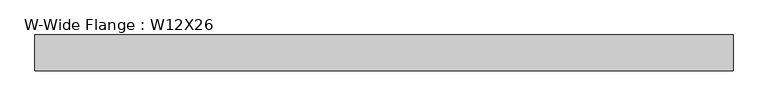
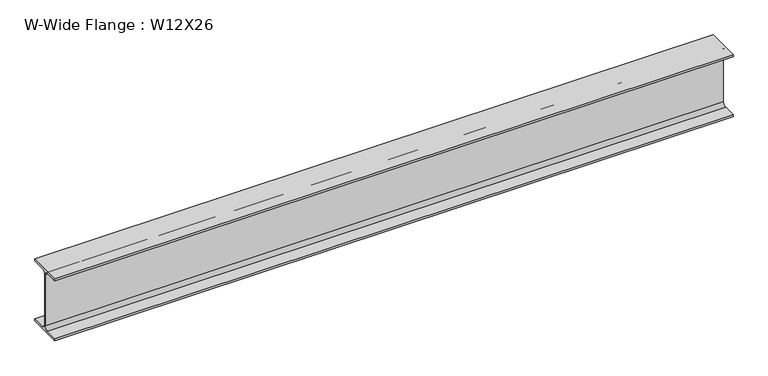
"""IFC4 building model written with IfcOpenShell, lengths in millimetres: beam geometry, W-Wide Flange : W12X26."""

from ifc_helpers import new_model, si_unit, point, frame, frame_2d, origin, place, context, project, spatial, polyline, circle_curve, trimmed, segment, composite_curve, outline, extrude, source, transform, mapped, element, save


def w_wide_flange_w12x26_2e5261f2(model_context):
    return source(origin(), model_context, "Body", "SweptSolid", [
        extrude(outline(composite_curve([segment(polyline([(82.4011719, -145.5539063), (82.4011719, -155.178125), (-82.4011719, -155.178125), (-82.4011719, -145.5539063), (-20.2902344, -145.5539063)]), True, "CONTINUOUS"), segment(trimmed(circle_curve(frame_2d((-20.2902344, -128.190625)), 17.3632812), [point((-20.2902344, -145.5539063))], [point((-2.9269531, -128.190625))], True, "CARTESIAN"), True, "CONTINUOUS"), segment(polyline([(-2.9269531, -128.190625), (-2.9269531, 128.190625)]), True, "CONTINUOUS"), segment(trimmed(circle_curve(frame_2d((-20.2902344, 128.190625)), 17.3632812), [point((-2.9269531, 128.190625))], [point((-20.2902344, 145.5539062))], True, "CARTESIAN"), True, "CONTINUOUS"), segment(polyline([(-20.2902344, 145.5539062), (-82.4011719, 145.5539062), (-82.4011719, 155.178125), (82.4011719, 155.178125), (82.4011719, 145.5539062), (20.2902344, 145.5539062)]), True, "CONTINUOUS"), segment(trimmed(circle_curve(frame_2d((20.2902344, 128.190625)), 17.3632812), [point((20.2902344, 145.5539062))], [point((2.9269531, 128.190625))], True, "CARTESIAN"), True, "CONTINUOUS"), segment(polyline([(2.9269531, 128.190625), (2.9269531, -128.190625)]), True, "CONTINUOUS"), segment(trimmed(circle_curve(frame_2d((20.2902344, -128.190625)), 17.3632812), [point((2.9269531, -128.190625))], [point((20.2902344, -145.5539063))], True, "CARTESIAN"), True, "CONTINUOUS"), segment(polyline([(20.2902344, -145.5539063), (82.4011719, -145.5539063)]), True, "CONTINUOUS")], self_intersect=False)), frame((-1609.7994141, 0.0, 0.0), z_axis=(1.0, 0.0, 0.0), x_axis=(0.0, 1.0, 0.0)), (0.0, 0.0, 1.0), 3219.5988281),
    ])


if __name__ == "__main__":
    model = new_model("IFC4")
    model_context = context("Model", 3, world=origin())
    ifc_project = project(units=[si_unit("LENGTHUNIT", "METRE", prefix="MILLI")], contexts=[model_context])
    site = spatial("IfcSite", under=ifc_project)
    building = spatial("IfcBuilding", under=site)
    placement = place(None, origin())
    w_wide_flange_w12x26_shape = w_wide_flange_w12x26_2e5261f2(model_context)
    element("IfcBeam", 1, ObjectType="W-Wide Flange : W12X26", at=placement, inside=building, context=model_context, shape_type="MappedRepresentation", body=[
        mapped(w_wide_flange_w12x26_shape, transform((0.0, 0.0, 0.0), x_axis=(1.0, 0.0, 0.0), y_axis=(0.0, 1.0, 0.0), z_axis=(0.0, 0.0, 1.0))),
    ])
    save(model, "model.ifc")

# Revit data of these elements
# Type "W-Wide Flange : W12X26"
#   Assembly Code = "B10"
#   W = 26
#   Length [instance default] = 5' - 0"
#   bf = 0' - 6 125/256"
#   d = 1' - 0 7/32"
#   k = 0' - 1 1/16"
#   k2 = 0' - 0 175/256"
#   tf = 0' - 0 97/256"
#   tw = 0' - 0 59/256"
#   A = 0.053125 SF
#   Structural Material [instance default] = none
# Element 1 (IfcBeam, "W-Wide Flange : W12X26")
#   Structural Material = Dark metal
#   Materials on its faces: "Dark metal"
# Materials
#   "Dark metal": class "Generic", colour RGB 44 29 29, transparency 0, Cost = 0
